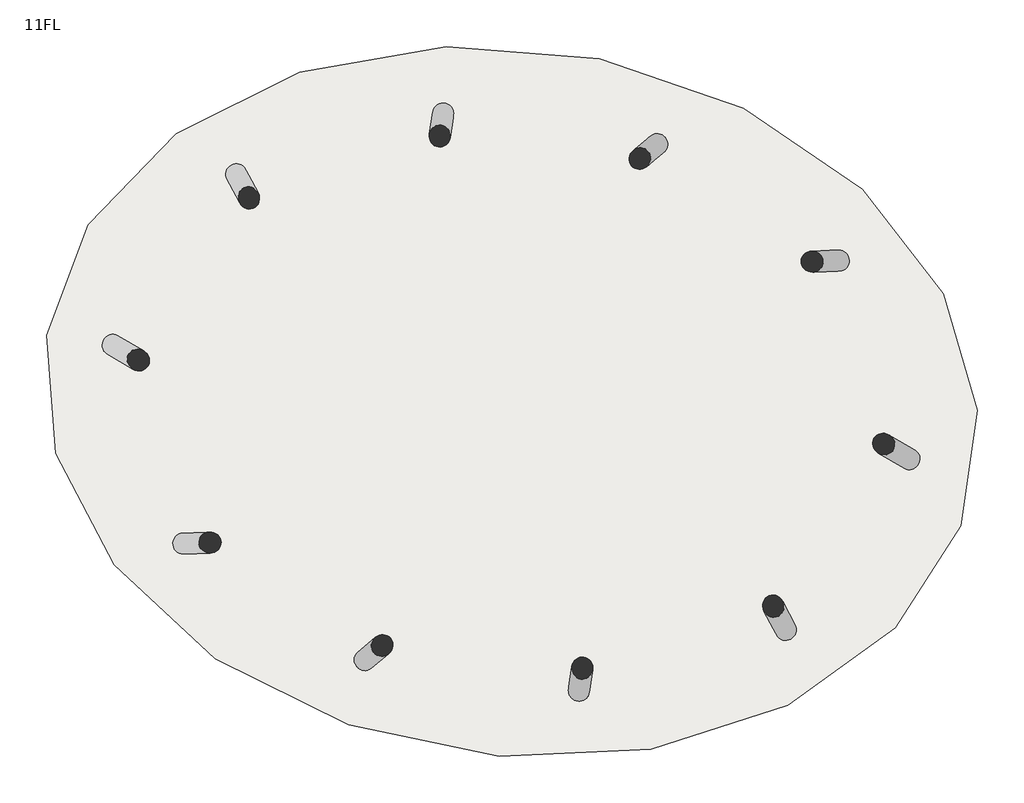
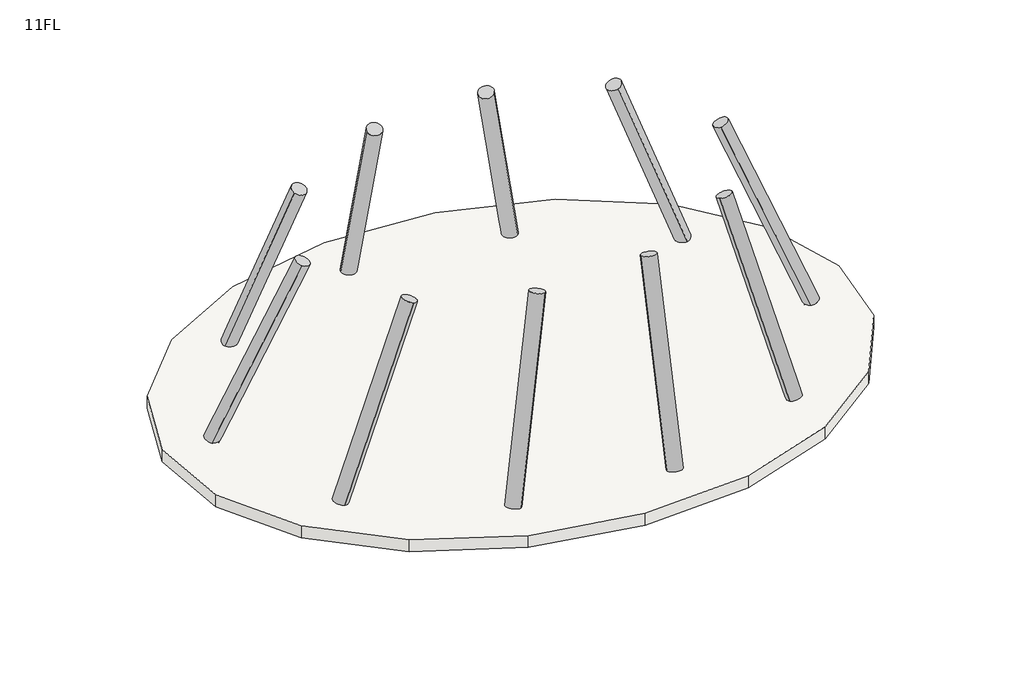
# One storey: 10 columns, 1 slab.
"""IFC4 building model written with IfcOpenShell, lengths in millimetres."""

from ifc_helpers import new_model, si_unit, point, frame, frame_2d, origin, place, context, project, spatial, polyline, circle_curve, trimmed, segment, composite_curve, outline, extrude, element, save

model = new_model("IFC4")

# Units and contexts
model_context = context("Model", 3, world=origin())
ifc_project = project(units=[si_unit("LENGTHUNIT", "METRE", prefix="MILLI")], contexts=[model_context])

# Site, building, storey
site = spatial("IfcSite", under=ifc_project)
building = spatial("IfcBuilding", under=site)
storey = spatial("IfcBuildingStorey", under=building, Name="11FL", Elevation=45000.0)

# Columns
placement = place(None, origin())
element("IfcColumn", 1, ObjectType="コンクリート-円形-柱 : 750", at=placement, inside=storey, context=model_context, shape_type="SweptSolid", body=[
    extrude(outline(composite_curve([segment(trimmed(circle_curve(frame_2d((0.0, -175.0)), 175.0), [point((0.0, -350.0))], [point((0.0, 0.0))], False, "CARTESIAN"), True, "CONTINUOUS"), segment(trimmed(circle_curve(frame_2d((0.0, -175.0)), 175.0), [point((0.0, 0.0))], [point((0.0, -350.0))], False, "CARTESIAN"), True, "CONTINUOUS")], self_intersect=False)), frame((-6533.7168646, 1103.0683448, 45000.0), z_axis=(0.3326193292008433, -0.19521767954583416, 0.9226345102123163), x_axis=(0.7957106520636333, -0.467010703974961, -0.3856754601543622)), (0.0, 0.0, 1.0), 4877.3376133),
])
element("IfcColumn", 2, ObjectType="コンクリート-円形-柱 : 750", at=placement, inside=storey, context=model_context, shape_type="SweptSolid", body=[
    extrude(outline(composite_curve([segment(trimmed(circle_curve(frame_2d((0.0, -175.0)), 175.0), [point((-1e-07, -350.0))], [point((0.0, 0.0))], False, "CARTESIAN"), True, "CONTINUOUS"), segment(trimmed(circle_curve(frame_2d((0.0, -175.0)), 175.0), [point((0.0, 0.0))], [point((-1e-07, -350.0))], False, "CARTESIAN"), True, "CONTINUOUS")], self_intersect=False)), frame((-5458.0163963, -2175.7080934, 45000.0), z_axis=(0.35070991788514877, 0.013415528457330583, 0.9363880483502568), x_axis=(0.9357037128846163, 0.0357929991359535, -0.35096641279016605)), (0.0, 0.0, 1.0), 4805.6999531),
])
element("IfcColumn", 3, ObjectType="コンクリート-円形-柱 : 750", at=placement, inside=storey, context=model_context, shape_type="SweptSolid", body=[
    extrude(outline(composite_curve([segment(trimmed(circle_curve(frame_2d((0.0, -175.0)), 175.0), [point((0.0, -350.0))], [point((0.0, 0.0))], False, "CARTESIAN"), True, "CONTINUOUS"), segment(trimmed(circle_curve(frame_2d((0.0, -175.0)), 175.0), [point((0.0, 0.0))], [point((0.0, -350.0))], False, "CARTESIAN"), True, "CONTINUOUS")], self_intersect=False)), frame((-2545.8827485, -4152.6671476, 45000.0), z_axis=(0.23264885021192128, 0.19412294994660845, 0.9529904473808211), x_axis=(0.7317223817124671, 0.6105515120775087, -0.3030003419154877)), (0.0, 0.0, 1.0), 4721.9780769),
])
element("IfcColumn", 4, ObjectType="コンクリート-円形-柱 : 750", at=placement, inside=storey, context=model_context, shape_type="SweptSolid", body=[
    extrude(outline(composite_curve([segment(trimmed(circle_curve(frame_2d((0.0, -175.0)), 175.0), [point((0.0, -350.0))], [point((0.0, 0.0))], False, "CARTESIAN"), True, "CONTINUOUS"), segment(trimmed(circle_curve(frame_2d((0.0, -175.0)), 175.0), [point((0.0, 0.0))], [point((0.0, -350.0))], False, "CARTESIAN"), True, "CONTINUOUS")], self_intersect=False)), frame((954.2062944, -4773.859981, 45000.0), z_axis=(0.04397439875913128, 0.30230351660406835, 0.9521968473496364), x_axis=(0.1370681578891589, 0.9422797653539311, -0.3054851287663825)), (0.0, 0.0, 1.0), 4725.9135677),
])
element("IfcColumn", 5, ObjectType="コンクリート-円形-柱 : 750", at=placement, inside=storey, context=model_context, shape_type="SweptSolid", body=[
    extrude(outline(composite_curve([segment(trimmed(circle_curve(frame_2d((0.0, -175.0)), 175.0), [point((1e-07, -350.0))], [point((0.0, 0.0))], False, "CARTESIAN"), True, "CONTINUOUS"), segment(trimmed(circle_curve(frame_2d((0.0, -175.0)), 175.0), [point((0.0, 0.0))], [point((1e-07, -350.0))], False, "CARTESIAN"), True, "CONTINUOUS")], self_intersect=False)), frame((4413.8483819, -3873.5064307, 45000.0), z_axis=(-0.1667271410889405, 0.31274999674160064, 0.9350879637565854), x_axis=(-0.4398917306589946, 0.8251574184725433, -0.35441571640879965)), (0.0, 0.0, 1.0), 4812.3814891),
])
element("IfcColumn", 6, ObjectType="コンクリート-円形-柱 : 750", at=placement, inside=storey, context=model_context, shape_type="SweptSolid", body=[
    extrude(outline(composite_curve([segment(trimmed(circle_curve(frame_2d((0.0, -174.9999999)), 175.0), [point((0.0, -349.9999999))], [point((0.0, 0.0))], False, "CARTESIAN"), True, "CONTINUOUS"), segment(trimmed(circle_curve(frame_2d((0.0, -174.9999999)), 175.0), [point((0.0, 0.0))], [point((0.0, -349.9999999))], False, "CARTESIAN"), True, "CONTINUOUS")], self_intersect=False)), frame((6533.7168823, -1103.0683146, 45000.0), z_axis=(-0.3326193307958236, 0.19521767322114614, 0.9226345109755327), x_axis=(-0.7957106603043957, 0.46701069144185875, -0.3856754583285534)), (0.0, 0.0, 1.0), 4877.3376133),
])
element("IfcColumn", 7, ObjectType="コンクリート-円形-柱 : 750", at=placement, inside=storey, context=model_context, shape_type="SweptSolid", body=[
    extrude(outline(composite_curve([segment(trimmed(circle_curve(frame_2d((-1e-07, -175.0)), 175.0), [point((0.0, -349.9999999))], [point((0.0, 0.0))], False, "CARTESIAN"), True, "CONTINUOUS"), segment(trimmed(circle_curve(frame_2d((-1e-07, -175.0)), 175.0), [point((0.0, 0.0))], [point((0.0, -349.9999999))], False, "CARTESIAN"), True, "CONTINUOUS")], self_intersect=False)), frame((5458.0163693, 2175.7081126, 45000.0), z_axis=(-0.3507099166195897, -0.013415525545592498, 0.9363880488659688), x_axis=(-0.935703713691752, -0.0357929915273924, -0.35096641141423207)), (0.0, 0.0, 1.0), 4805.6999531),
])
element("IfcColumn", 8, ObjectType="コンクリート-円形-柱 : 750", at=placement, inside=storey, context=model_context, shape_type="SweptSolid", body=[
    extrude(outline(composite_curve([segment(trimmed(circle_curve(frame_2d((0.0, -175.0)), 175.0), [point((0.0, -350.0))], [point((0.0, 0.0))], False, "CARTESIAN"), True, "CONTINUOUS"), segment(trimmed(circle_curve(frame_2d((0.0, -175.0)), 175.0), [point((0.0, 0.0))], [point((0.0, -350.0))], False, "CARTESIAN"), True, "CONTINUOUS")], self_intersect=False)), frame((2545.8827139, 4152.66714, 45000.0), z_axis=(-0.2326488506445159, -0.19412294853879375, 0.9529904475619839), x_axis=(-0.7317223845881531, -0.6105515089138817, -0.303000341345698)), (0.0, 0.0, 1.0), 4721.9780769),
])
element("IfcColumn", 9, ObjectType="コンクリート-円形-柱 : 750", at=placement, inside=storey, context=model_context, shape_type="SweptSolid", body=[
    extrude(outline(composite_curve([segment(trimmed(circle_curve(frame_2d((0.0, -174.9999999)), 175.0), [point((0.0, -350.0))], [point((0.0, 0.0))], False, "CARTESIAN"), True, "CONTINUOUS"), segment(trimmed(circle_curve(frame_2d((0.0, -174.9999999)), 175.0), [point((0.0, 0.0))], [point((0.0, -350.0))], False, "CARTESIAN"), True, "CONTINUOUS")], self_intersect=False)), frame((-954.2063231, 4773.8599795, 45000.0), z_axis=(-0.04397440001869516, -0.3023035174066518, 0.9521968470366629), x_axis=(-0.13706816133245167, -0.9422797645367872, -0.3054851297419206)), (0.0, 0.0, 1.0), 4725.9135677),
])
element("IfcColumn", 10, ObjectType="コンクリート-円形-柱 : 750", at=placement, inside=storey, context=model_context, shape_type="SweptSolid", body=[
    extrude(outline(composite_curve([segment(trimmed(circle_curve(frame_2d((0.0, -175.0)), 175.0), [point((0.0, -349.9999999))], [point((0.0, 0.0))], False, "CARTESIAN"), True, "CONTINUOUS"), segment(trimmed(circle_curve(frame_2d((0.0, -175.0)), 175.0), [point((0.0, 0.0))], [point((0.0, -349.9999999))], False, "CARTESIAN"), True, "CONTINUOUS")], self_intersect=False)), frame((-4413.8484069, 3873.506424, 45000.0), z_axis=(0.16672714255269028, -0.3127500015216601, 0.9350879618968562), x_axis=(0.4398917275560064, -0.8251574180192582, -0.35441572131549626)), (0.0, 0.0, 1.0), 4812.3814891),
])

# Slab
element("IfcSlab", 11, ObjectType="一般 300 mm", at=placement, inside=storey, context=model_context, shape_type="SweptSolid", body=[
    extrude(outline(polyline([(-6591.8020747, -2704.5669986), (-7564.3443375, -846.7172459), (-7713.5207453, 1109.0368535), (-7019.3874272, 2943.5413191), (-5562.8231985, 4452.1382845), (-3507.8658603, 5474.0300463), (-1077.6909263, 5903.7766851), (1467.2199751, 5697.8715888), (3854.6574912, 4878.8075737), (5828.7575054, 3532.8419101), (7175.9048629, 1801.1189564), (7745.4896351, -132.4995404), (7469.072302, -2055.0242169), (6377.7964544, -3749.8470119), (4597.3352881, -5031.8877458), (2323.9978524, -5767.1641123), (-197.488675, -5880.4313862), (-2697.3229734, -5361.0116303), (-4907.9851265, -4264.0133488), (-6591.8020747, -2704.5669986)])), frame((0.0, 0.0, 44700.0), z_axis=(0.0, 0.0, 1.0), x_axis=(1.0, 0.0, 0.0)), (0.0, 0.0, 1.0), 300.0),
])

save(model, "model.ifc")

# Revit data of these elements
# Type "コンクリート-円形-柱 : 750"
#   Keynote = "03310.Q1"
#   R = 350 mm
#   Structural Material [instance default] = コンクリート - 現場打ち
# Type "一般 300 mm"
#   Function = 0
#   Layers, outside or top first: 300 mm no material (function 1)
# Elements 1, 2, 3, 4, 5, 6, 7, 8, 9, 10 (IfcColumn, "コンクリート-円形-柱 : 750")
#   Structural Material = コンクリート - 現場打ち
#   Phase Created = 新しい建設
#   Materials on its faces: "コンクリート - 現場打ち"
# Element 11 (IfcSlab, "一般 300 mm")
#   Height Offset From Level = 0 mm
#   Phase Created = 新しい建設
# Materials
#   "コンクリート - 現場打ち": class "コンクリート", colour RGB 192 192 192, transparency 0
